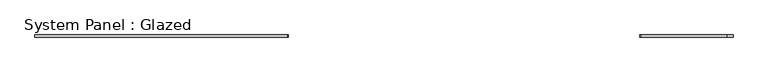
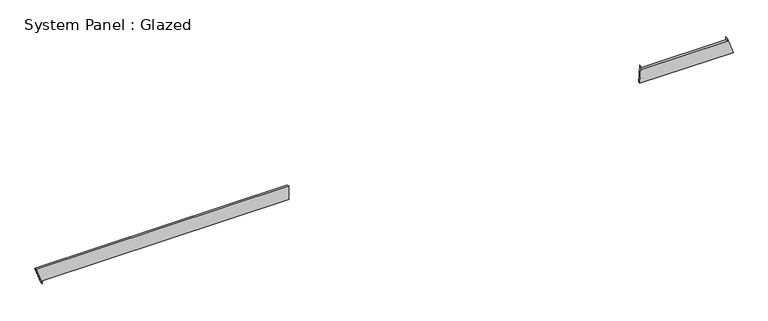
"""IFC4 building model written with IfcOpenShell, lengths in millimetres: plate geometry, System Panel : Glazed."""

from ifc_helpers import new_model, si_unit, frame, origin, place, context, project, spatial, polyline, outline, extrude, source, transform, mapped, element, save


def system_panel_glazed_8638838d(model_context):
    return source(origin(), model_context, "Body", "SweptSolid", [
        extrude(outline(polyline([(35.3553391, 2951.0791667), (35.3553391, 4027.3165452), (235.5515472, 3958.146555), (200.1962081, 3958.1472368), (200.1769629, 2960.261132), (235.5323019, 2960.2604501), (35.3553391, 2951.0791667)])), frame((0.0, -49.5, 0.0), z_axis=(0.0, 1.0, 0.0), x_axis=(0.0, 0.0, 1.0)), (0.0, 0.0, 1.0), 25.0),
        extrude(outline(polyline([(0.0, -3957.7762608), (35.3553391, -3957.7762608), (35.3553391, -1106.9063958), (200.0984696, -1109.6990095), (200.0422004, -4027.3165452), (0.0, -3957.7762608)])), frame((0.0, -49.5, 0.0), z_axis=(0.0, 1.0, 0.0), x_axis=(0.0, 0.0, 1.0)), (0.0, 0.0, 1.0), 25.0),
    ])


if __name__ == "__main__":
    model = new_model("IFC4")
    model_context = context("Model", 3, world=origin())
    ifc_project = project(units=[si_unit("LENGTHUNIT", "METRE", prefix="MILLI")], contexts=[model_context])
    site = spatial("IfcSite", under=ifc_project)
    building = spatial("IfcBuilding", under=site)
    placement = place(None, origin())
    system_panel_glazed_shape = system_panel_glazed_8638838d(model_context)
    element("IfcPlate", 1, ObjectType="System Panel : Glazed", at=placement, inside=building, context=model_context, shape_type="MappedRepresentation", body=[
        mapped(system_panel_glazed_shape, transform((0.0, 0.0, 0.0), x_axis=(1.0, 0.0, 0.0), y_axis=(0.0, 1.0, 0.0), z_axis=(0.0, 0.0, 1.0))),
    ])
    save(model, "model.ifc")

# Revit data of these elements
# Element 1 (IfcPlate, "System Panel : Glazed")
#   Materials on its faces: "Glass"
# Materials
#   "Glass": class "Glass", colour RGB 218 227 224, transparency 0.85, Description = "Soda Lime Glass", Cost = 0
